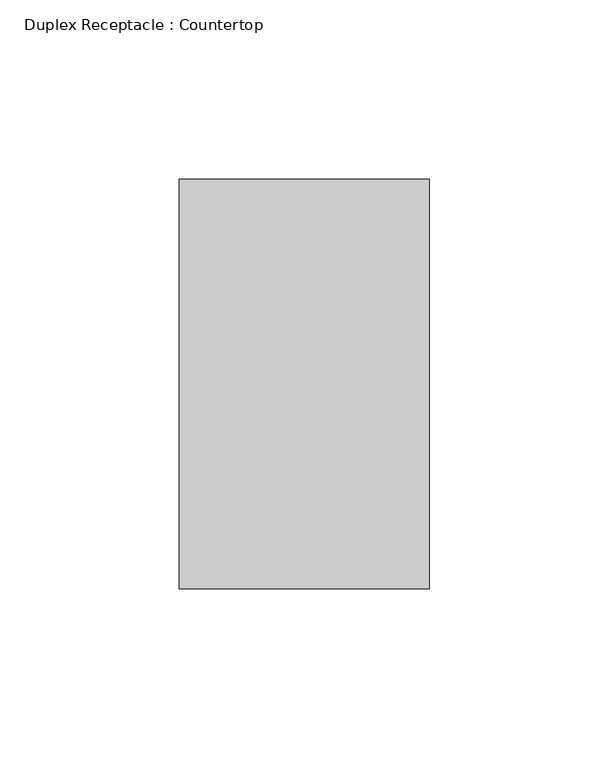
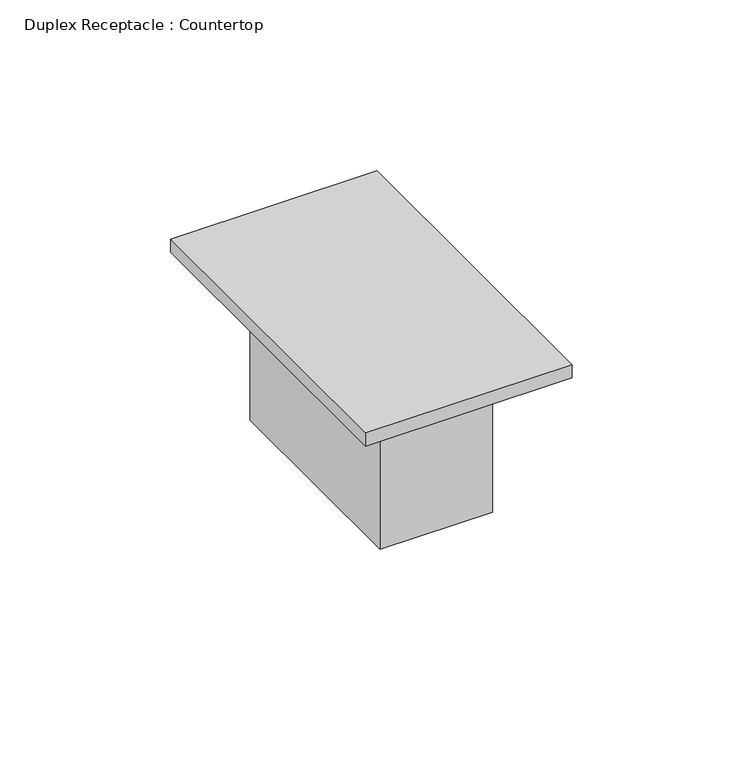
"""IFC4 building model written with IfcOpenShell, lengths in millimetres: proxy geometry, Duplex Receptacle : Countertop."""

import ifcopenshell
import ifcopenshell.guid

model = None  # the IFC model being written
_history = None  # IfcOwnerHistory: only IFC2X3 demands one
_inside = {}  # id of a spatial element -> (the spatial element, [elements in it])
_under = {}  # id of a project, library or spatial element -> (it, [spatial elements below it])
_declared = {}  # id of a project -> (the project, [libraries it declares])
_typed = {}  # id of a type object -> (the type object, [elements of that type])
_made_of = {}  # id of a material, layer set ... -> (it, [elements and type objects made of it])


def new_model(schema):
    """Start an empty IFC model of exactly this schema.

    Asked for "IFC4X3", IfcOpenShell would pick the latest addendum, in which some entities
    have other attributes; the version numbers below select the first issue.
    IFC2X3 requires an IfcOwnerHistory on every rooted entity: one is made here for all.
    """
    global model, _history
    if schema == "IFC4X3":
        model = ifcopenshell.file(schema_version=(4, 3, 0, 0))
    else:
        model = ifcopenshell.file(schema=schema)
    _inside.clear()
    _under.clear()
    _declared.clear()
    _typed.clear()
    _made_of.clear()
    _history = None
    if model.schema == "IFC2X3":
        org = make("IfcOrganization", Name="unknown")
        user = make(
            "IfcPersonAndOrganization",
            ThePerson=make("IfcPerson", FamilyName="unknown"),
            TheOrganization=org,
        )
        app = make(
            "IfcApplication",
            ApplicationDeveloper=org,
            Version="unknown",
            ApplicationFullName="unknown",
            ApplicationIdentifier="unknown",
        )
        _history = make(
            "IfcOwnerHistory",
            OwningUser=user,
            OwningApplication=app,
            ChangeAction="ADDED",
            CreationDate=0,
        )
    return model


def make(cls, **values):
    """One entity of the class cls with the attributes given. An attribute that is None is left unset."""
    return model.create_entity(
        cls, **{name: value for name, value in values.items() if value is not None}
    )


def rooted(cls, **values):
    """An entity with a GlobalId (a new one), such as an element, a storey or a relation."""
    return make(cls, GlobalId=ifcopenshell.guid.new(), OwnerHistory=_history, **values)


def si_unit(unit_type, name, prefix=None):
    """IfcSIUnit, for example si_unit("LENGTHUNIT", "METRE", prefix="MILLI")."""
    return make("IfcSIUnit", UnitType=unit_type, Prefix=prefix, Name=name)


def assignment(units):
    """IfcUnitAssignment: the units of a project."""
    return None if units is None else make("IfcUnitAssignment", Units=units)


def point(xyz):
    """IfcCartesianPoint."""
    return None if xyz is None else make("IfcCartesianPoint", Coordinates=xyz)


def direction(xyz):
    """IfcDirection."""
    return None if xyz is None else make("IfcDirection", DirectionRatios=xyz)


def frame(location, z_axis=None, x_axis=None):
    """IfcAxis2Placement3D, a coordinate frame: its origin and axes. An axis left out is left unset."""
    return make(
        "IfcAxis2Placement3D",
        Location=point(location),
        Axis=direction(z_axis),
        RefDirection=direction(x_axis),
    )


def origin():
    """The frame at (0, 0, 0) with its axes left unset."""
    return frame((0.0, 0.0, 0.0))


def origin_with_axes():
    """The frame at (0, 0, 0) with the z axis (0, 0, 1) and the x axis (1, 0, 0) written out."""
    return frame((0.0, 0.0, 0.0), z_axis=(0.0, 0.0, 1.0), x_axis=(1.0, 0.0, 0.0))


def place(relative_to, where):
    """IfcLocalPlacement: puts the frame where relative to a parent placement (None: the world)."""
    return make(
        "IfcLocalPlacement", PlacementRelTo=relative_to, RelativePlacement=where
    )


def context(
    kind, dimensions, precision=None, world=None, true_north=None, identifier=None
):
    """IfcGeometricRepresentationContext, for example the 3D "Model" context."""
    return make(
        "IfcGeometricRepresentationContext",
        ContextIdentifier=identifier,
        ContextType=kind,
        CoordinateSpaceDimension=dimensions,
        Precision=precision,
        WorldCoordinateSystem=world,
        TrueNorth=true_north,
    )


def project(units=None, contexts=None):
    """IfcProject with its units and contexts."""
    return rooted(
        "IfcProject",
        Name="project",
        RepresentationContexts=contexts,
        UnitsInContext=assignment(units),
    )


def spatial(cls, under=None, at=None, **own):
    """A site, building, storey or space (cls), placed at a placement, below another one or the project."""
    s = rooted(cls, ObjectPlacement=at, **own)
    if under is not None:
        _under.setdefault(under.id(), (under, []))[1].append(s)
    return s


def polyline(points):
    """IfcPolyline through the points."""
    return make("IfcPolyline", Points=[point(p) for p in points])


def outline(outer, holes=None, kind="AREA"):
    """IfcArbitraryClosedProfileDef: a profile drawn as a closed curve; with holes, ...WithVoids."""
    if holes is None:
        return make("IfcArbitraryClosedProfileDef", ProfileType=kind, OuterCurve=outer)
    return make(
        "IfcArbitraryProfileDefWithVoids",
        ProfileType=kind,
        OuterCurve=outer,
        InnerCurves=holes,
    )


def extrude(swept, where, along, depth):
    """IfcExtrudedAreaSolid: the profile swept, set in the frame where, extruded along a direction by depth."""
    return make(
        "IfcExtrudedAreaSolid",
        SweptArea=swept,
        Position=where,
        ExtrudedDirection=direction(along),
        Depth=depth,
    )


def shape(context_of_items, identifier, shape_type, items):
    """IfcShapeRepresentation: the items that make up one representation, for example the "Body"."""
    return make(
        "IfcShapeRepresentation",
        ContextOfItems=context_of_items,
        RepresentationIdentifier=identifier,
        RepresentationType=shape_type,
        Items=items,
    )


def source(mapping_origin, context_of_items, identifier, shape_type, items):
    """IfcRepresentationMap: a shape defined once, which mapped items show again and again."""
    return make(
        "IfcRepresentationMap",
        MappingOrigin=mapping_origin,
        MappedRepresentation=shape(context_of_items, identifier, shape_type, items),
    )


def transform(
    local_origin,
    x_axis=None,
    y_axis=None,
    z_axis=None,
    scale=None,
    scale2=None,
    scale3=None,
    uniform=True,
):
    """IfcCartesianTransformationOperator3D, or its non-uniform kind. x_axis, y_axis, z_axis: its Axis1, 2, 3."""
    if uniform:
        return make(
            "IfcCartesianTransformationOperator3D",
            Axis1=direction(x_axis),
            Axis2=direction(y_axis),
            LocalOrigin=point(local_origin),
            Scale=scale,
            Axis3=direction(z_axis),
        )
    return make(
        "IfcCartesianTransformationOperator3DnonUniform",
        Axis1=direction(x_axis),
        Axis2=direction(y_axis),
        LocalOrigin=point(local_origin),
        Scale=scale,
        Axis3=direction(z_axis),
        Scale2=scale2,
        Scale3=scale3,
    )


def mapped(mapping_source, mapping_target):
    """IfcMappedItem: shows the shape of a source again, moved by a transform."""
    return make(
        "IfcMappedItem", MappingSource=mapping_source, MappingTarget=mapping_target
    )


def made_of(thing, what):
    """Note that an element or type object is made of a material, layer set ...; save() writes the relation."""
    if what is not None:
        _made_of.setdefault(what.id(), (what, []))[1].append(thing)
    return thing


def element(
    cls,
    number,
    at=None,
    inside=None,
    cuts=None,
    type_object=None,
    material=None,
    context=None,
    identifier="Body",
    shape_type=None,
    held_by="IfcProductDefinitionShape",
    body=None,
    shapes=None,
    **own,
):
    """One element of the class cls, such as IfcWall. Its Tag is "e" and its number.

    at: its placement. inside: the storey or other place that contains it. cuts: it is an
    opening in that element (IfcRelVoidsElement). A single representation is given by context,
    identifier, shape_type and body (its items); several are given by shapes. held_by: the class
    of the entity that holds the representations. save() writes the other relations.
    """
    e = rooted(cls, Tag="e%d" % number, ObjectPlacement=at, **own)
    if body is not None:
        shapes = [shape(context, identifier, shape_type, body)]
    if shapes is not None:
        e.Representation = make(held_by, Representations=shapes)
    if inside is not None:
        _inside.setdefault(inside.id(), (inside, []))[1].append(e)
    if cuts is not None:
        rooted(
            "IfcRelVoidsElement", RelatingBuildingElement=cuts, RelatedOpeningElement=e
        )
    if type_object is not None:
        _typed.setdefault(type_object.id(), (type_object, []))[1].append(e)
    return made_of(e, material)


def aggregate(whole, parts):
    """IfcRelAggregates: a whole, such as a stair, and the parts it consists of."""
    return rooted("IfcRelAggregates", RelatingObject=whole, RelatedObjects=parts)


def save(model, path):
    """Write the relations noted so far, then the file.

    IfcRelAggregates (storeys below a building ...), IfcRelContainedInSpatialStructure (elements
    in a storey), IfcRelDefinesByType, IfcRelAssociatesMaterial and IfcRelDeclares: one each for
    every whole, place, type object, material and project.
    """
    for whole, parts in _under.values():
        aggregate(whole, parts)
    for where, things in _inside.values():
        rooted(
            "IfcRelContainedInSpatialStructure",
            RelatedElements=things,
            RelatingStructure=where,
        )
    for kind, things in _typed.values():
        rooted("IfcRelDefinesByType", RelatedObjects=things, RelatingType=kind)
    for what, things in _made_of.values():
        rooted("IfcRelAssociatesMaterial", RelatedObjects=things, RelatingMaterial=what)
    for by, libraries in _declared.values():
        rooted("IfcRelDeclares", RelatingContext=by, RelatedDefinitions=libraries)
    model.write(path)


def duplex_receptacle_countertop_10251bba(model_context):
    return source(origin(), model_context, "Body", "SweptSolid", [
        extrude(outline(polyline([(19.05, 38.1), (19.05, -38.1), (-19.05, -38.1), (-19.05, 38.1), (19.05, 38.1)])), frame((0.0, 0.0, -53.975), z_axis=(0.0, 0.0, 1.0), x_axis=(1.0, 0.0, 0.0)), (0.0, 0.0, 1.0), 53.975),
        extrude(outline(polyline([(34.925, 57.15), (34.925, -57.15), (-34.925, -57.15), (-34.925, 57.15), (34.925, 57.15)])), origin_with_axes(), (0.0, 0.0, 1.0), 4.7625),
    ])


if __name__ == "__main__":
    model = new_model("IFC4")
    model_context = context("Model", 3, world=origin())
    ifc_project = project(units=[si_unit("LENGTHUNIT", "METRE", prefix="MILLI")], contexts=[model_context])
    site = spatial("IfcSite", under=ifc_project)
    building = spatial("IfcBuilding", under=site)
    placement = place(None, origin())
    duplex_receptacle_countertop_shape = duplex_receptacle_countertop_10251bba(model_context)
    element("IfcBuildingElementProxy", 1, Name="Duplex Receptacle : Countertop", ObjectType="Duplex Receptacle : Countertop", at=placement, inside=building, context=model_context, shape_type="MappedRepresentation", body=[
        mapped(duplex_receptacle_countertop_shape, transform((0.0, 0.0, 0.0), x_axis=(1.0, 0.0, 0.0), y_axis=(0.0, 1.0, 0.0), z_axis=(0.0, 0.0, 1.0))),
    ])
    save(model, "model.ifc")

# Revit data of these elements
# Project information
#   Project Issue Date = "Issue Date"
#   Project Status = "Project Status"
#   Client Name = "Owner"
#   Project Address = "Enter address here"
#   Project Name = "Project Name"
#   Project Number = "Project Number"
# Type "Duplex Receptacle : Countertop"
#   Label = "CTR"
#   Switch Voltage = 120 V
#   Load = 180 VA
#   Default Elevation = 1' - 6"
#   Load Classification = Receptacle
#   Assembly Code = ""
